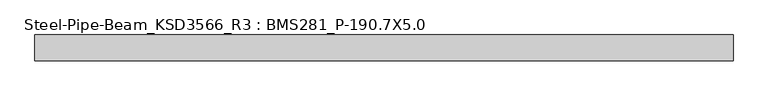
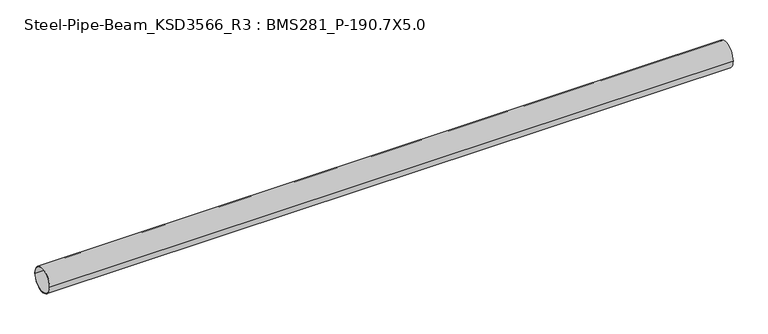
"""IFC4 building model written with IfcOpenShell, lengths in millimetres: member geometry, Steel-Pipe-Beam_KSD3566_R3 : BMS281_P-190.7X5.0."""

from ifc_helpers import new_model, si_unit, point, frame, origin, origin_2d, place, context, project, spatial, circle_curve, trimmed, segment, composite_curve, outline, extrude, source, transform, mapped, element, save


def steel_pipe_beam_ksd3566_r3_bms281_p_190_7x5_0_938622a6(model_context):
    return source(origin(), model_context, "Body", "SweptSolid", [
        extrude(outline(composite_curve([segment(trimmed(circle_curve(origin_2d(), 95.35), [point((-95.35, 0.0))], [point((95.35, 0.0))], False, "CARTESIAN"), True, "CONTINUOUS"), segment(trimmed(circle_curve(origin_2d(), 95.35), [point((95.35, 0.0))], [point((-95.35, 0.0))], False, "CARTESIAN"), True, "CONTINUOUS")], self_intersect=False), holes=[composite_curve([segment(trimmed(circle_curve(origin_2d(), 90.35), [point((90.35, 0.0))], [point((-90.35, 0.0))], True, "CARTESIAN"), True, "CONTINUOUS"), segment(trimmed(circle_curve(origin_2d(), 90.35), [point((-90.35, 0.0))], [point((90.35, 0.0))], True, "CARTESIAN"), True, "CONTINUOUS")], self_intersect=False)]), frame((-2577.1305565, 0.0, 0.0), z_axis=(1.0, 0.0, 0.0), x_axis=(0.0, 1.0, 0.0)), (0.0, 0.0, 1.0), 5164.9165514),
    ])


if __name__ == "__main__":
    model = new_model("IFC4")
    model_context = context("Model", 3, world=origin())
    ifc_project = project(units=[si_unit("LENGTHUNIT", "METRE", prefix="MILLI")], contexts=[model_context])
    site = spatial("IfcSite", under=ifc_project)
    building = spatial("IfcBuilding", under=site)
    placement = place(None, origin())
    steel_pipe_beam_ksd3566_r3_bms281_p_190_7x5_0_shape = steel_pipe_beam_ksd3566_r3_bms281_p_190_7x5_0_938622a6(model_context)
    element("IfcMember", 1, ObjectType="Steel-Pipe-Beam_KSD3566_R3 : BMS281_P-190.7X5.0", at=placement, inside=building, context=model_context, shape_type="MappedRepresentation", body=[
        mapped(steel_pipe_beam_ksd3566_r3_bms281_p_190_7x5_0_shape, transform((0.0, 0.0, 0.0), x_axis=(1.0, 0.0, 0.0), y_axis=(0.0, 1.0, 0.0), z_axis=(0.0, 0.0, 1.0))),
    ])
    save(model, "model.ifc")

# Revit data of these elements
# Type "Steel-Pipe-Beam_KSD3566_R3 : BMS281_P-190.7X5.0"
#   Keynote = "P-190.7X5.0"
#   SteelWeight = "Light"
#   t = 0.0050 m
#   Surface Area = 0.599102 m²/m
#   Section Area = 29.1697 cm²
#   Mass per Unit Length = 22.8982 kg/m
#   Length [instance default] = 1.5000 m
#   D = 0.1907 m
#   hec_material4 [instance default] = none
#   hec_material3 [instance default] = none
#   hec_material2 [instance default] = none
#   hec_material1 [instance default] = none
#   Structural Material [instance default] = Steel, 45-345
#   Assembly Code = ""
# Element 1 (IfcMember, "Steel-Pipe-Beam_KSD3566_R3 : BMS281_P-190.7X5.0")
#   Structural Material = none
# Materials
#   "Steel, 45-345": class "Metal", colour RGB 189 187 185, transparency 0, Description = "Steel 345 MPa", Cost = 0
